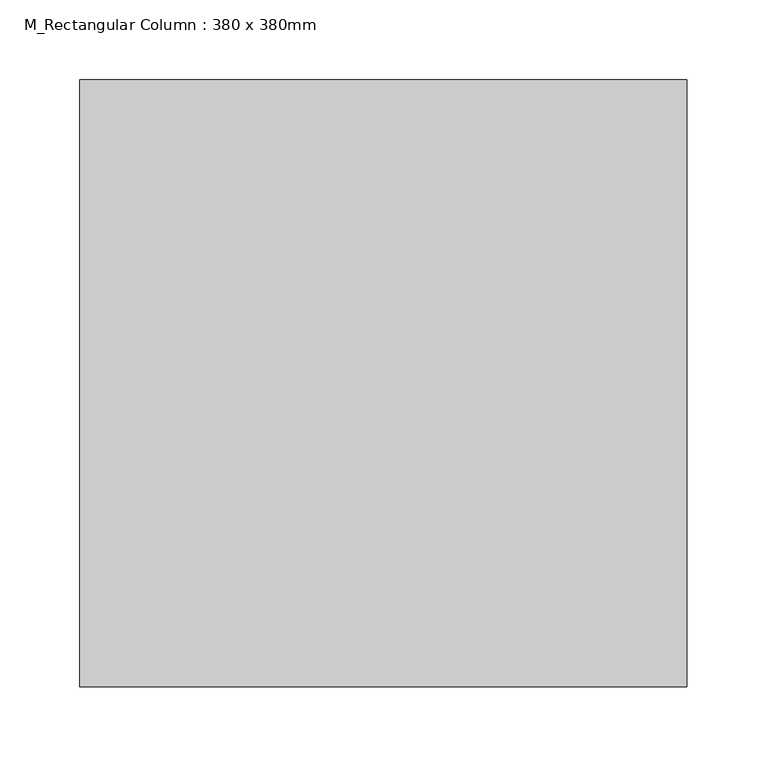
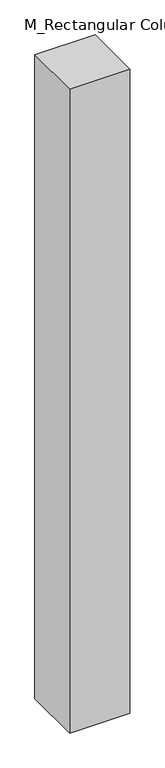
"""IFC4 building model written with IfcOpenShell, lengths in millimetres: column geometry, M_Rectangular Column : 380 x 380mm."""

from ifc_helpers import new_model, si_unit, origin, origin_with_axes, place, context, project, spatial, polyline, outline, extrude, source, transform, mapped, element, save


def m_rectangular_column_380_x_380mm_96b74405(model_context):
    return source(origin(), model_context, "Body", "SweptSolid", [
        extrude(outline(polyline([(190.0, 190.0), (190.0, -190.0), (-190.0, -190.0), (-190.0, 190.0), (190.0, 190.0)])), origin_with_axes(), (0.0, 0.0, 1.0), 4300.0),
    ])


if __name__ == "__main__":
    model = new_model("IFC4")
    model_context = context("Model", 3, world=origin())
    ifc_project = project(units=[si_unit("LENGTHUNIT", "METRE", prefix="MILLI")], contexts=[model_context])
    site = spatial("IfcSite", under=ifc_project)
    building = spatial("IfcBuilding", under=site)
    placement = place(None, origin())
    m_rectangular_column_380_x_380mm_shape = m_rectangular_column_380_x_380mm_96b74405(model_context)
    element("IfcColumn", 1, ObjectType="M_Rectangular Column : 380 x 380mm", at=placement, inside=building, context=model_context, shape_type="MappedRepresentation", body=[
        mapped(m_rectangular_column_380_x_380mm_shape, transform((0.0, 0.0, 0.0), x_axis=(1.0, 0.0, 0.0), y_axis=(0.0, 1.0, 0.0), z_axis=(0.0, 0.0, 1.0))),
    ])
    save(model, "model.ifc")

# Revit data of these elements
# Type "M_Rectangular Column : 380 x 380mm"
#   Depth = 38.0 cm
#   Offset Base = 0.0 cm
#   Offset Top = 0.0 cm
#   Width = 38.0 cm
#   Material = none
